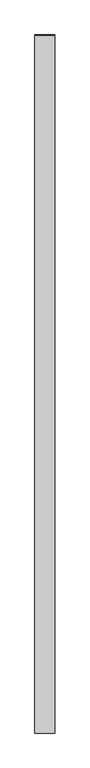
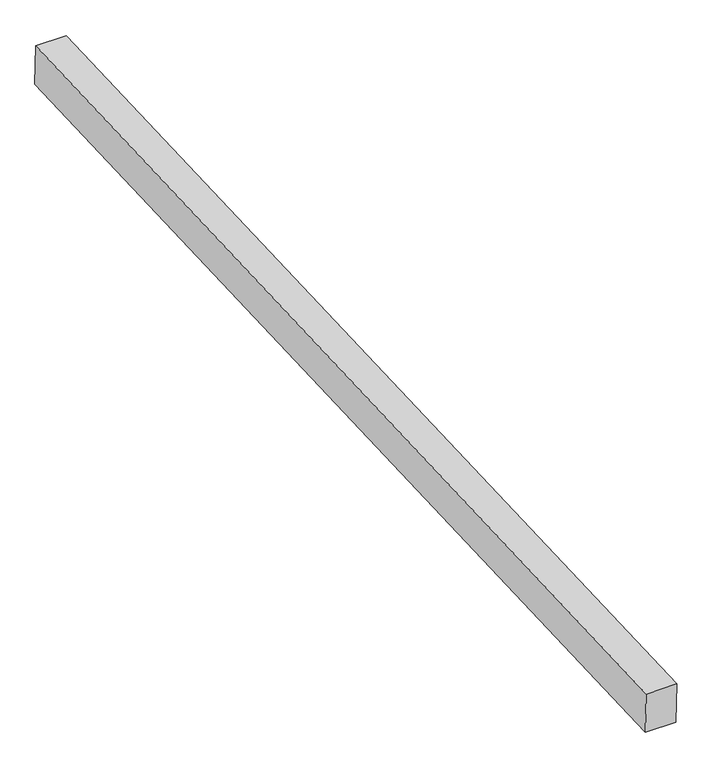
"""IFC4 building model written with IfcOpenShell, lengths in millimetres: proxy geometry, Generic Models 7:Generic Models 1:8:Generic Models 1:8 : Generic Models 7:Generic Models 1:337419:18 : Generic Models 7:Generic Models 1:8:Generic Models 1:8 : Generic Models 7:Generic Models 1:337419:315935."""

import ifcopenshell
import ifcopenshell.guid

model = None  # the IFC model being written
_history = None  # IfcOwnerHistory: only IFC2X3 demands one
_inside = {}  # id of a spatial element -> (the spatial element, [elements in it])
_under = {}  # id of a project, library or spatial element -> (it, [spatial elements below it])
_declared = {}  # id of a project -> (the project, [libraries it declares])
_typed = {}  # id of a type object -> (the type object, [elements of that type])
_made_of = {}  # id of a material, layer set ... -> (it, [elements and type objects made of it])


def new_model(schema):
    """Start an empty IFC model of exactly this schema.

    Asked for "IFC4X3", IfcOpenShell would pick the latest addendum, in which some entities
    have other attributes; the version numbers below select the first issue.
    IFC2X3 requires an IfcOwnerHistory on every rooted entity: one is made here for all.
    """
    global model, _history
    if schema == "IFC4X3":
        model = ifcopenshell.file(schema_version=(4, 3, 0, 0))
    else:
        model = ifcopenshell.file(schema=schema)
    _inside.clear()
    _under.clear()
    _declared.clear()
    _typed.clear()
    _made_of.clear()
    _history = None
    if model.schema == "IFC2X3":
        org = make("IfcOrganization", Name="unknown")
        user = make(
            "IfcPersonAndOrganization",
            ThePerson=make("IfcPerson", FamilyName="unknown"),
            TheOrganization=org,
        )
        app = make(
            "IfcApplication",
            ApplicationDeveloper=org,
            Version="unknown",
            ApplicationFullName="unknown",
            ApplicationIdentifier="unknown",
        )
        _history = make(
            "IfcOwnerHistory",
            OwningUser=user,
            OwningApplication=app,
            ChangeAction="ADDED",
            CreationDate=0,
        )
    return model


def make(cls, **values):
    """One entity of the class cls with the attributes given. An attribute that is None is left unset."""
    return model.create_entity(
        cls, **{name: value for name, value in values.items() if value is not None}
    )


def rooted(cls, **values):
    """An entity with a GlobalId (a new one), such as an element, a storey or a relation."""
    return make(cls, GlobalId=ifcopenshell.guid.new(), OwnerHistory=_history, **values)


def si_unit(unit_type, name, prefix=None):
    """IfcSIUnit, for example si_unit("LENGTHUNIT", "METRE", prefix="MILLI")."""
    return make("IfcSIUnit", UnitType=unit_type, Prefix=prefix, Name=name)


def assignment(units):
    """IfcUnitAssignment: the units of a project."""
    return None if units is None else make("IfcUnitAssignment", Units=units)


def point(xyz):
    """IfcCartesianPoint."""
    return None if xyz is None else make("IfcCartesianPoint", Coordinates=xyz)


def direction(xyz):
    """IfcDirection."""
    return None if xyz is None else make("IfcDirection", DirectionRatios=xyz)


def frame(location, z_axis=None, x_axis=None):
    """IfcAxis2Placement3D, a coordinate frame: its origin and axes. An axis left out is left unset."""
    return make(
        "IfcAxis2Placement3D",
        Location=point(location),
        Axis=direction(z_axis),
        RefDirection=direction(x_axis),
    )


def origin():
    """The frame at (0, 0, 0) with its axes left unset."""
    return frame((0.0, 0.0, 0.0))


def place(relative_to, where):
    """IfcLocalPlacement: puts the frame where relative to a parent placement (None: the world)."""
    return make(
        "IfcLocalPlacement", PlacementRelTo=relative_to, RelativePlacement=where
    )


def context(
    kind, dimensions, precision=None, world=None, true_north=None, identifier=None
):
    """IfcGeometricRepresentationContext, for example the 3D "Model" context."""
    return make(
        "IfcGeometricRepresentationContext",
        ContextIdentifier=identifier,
        ContextType=kind,
        CoordinateSpaceDimension=dimensions,
        Precision=precision,
        WorldCoordinateSystem=world,
        TrueNorth=true_north,
    )


def project(units=None, contexts=None):
    """IfcProject with its units and contexts."""
    return rooted(
        "IfcProject",
        Name="project",
        RepresentationContexts=contexts,
        UnitsInContext=assignment(units),
    )


def spatial(cls, under=None, at=None, **own):
    """A site, building, storey or space (cls), placed at a placement, below another one or the project."""
    s = rooted(cls, ObjectPlacement=at, **own)
    if under is not None:
        _under.setdefault(under.id(), (under, []))[1].append(s)
    return s


def polyline(points):
    """IfcPolyline through the points."""
    return make("IfcPolyline", Points=[point(p) for p in points])


def outline(outer, holes=None, kind="AREA"):
    """IfcArbitraryClosedProfileDef: a profile drawn as a closed curve; with holes, ...WithVoids."""
    if holes is None:
        return make("IfcArbitraryClosedProfileDef", ProfileType=kind, OuterCurve=outer)
    return make(
        "IfcArbitraryProfileDefWithVoids",
        ProfileType=kind,
        OuterCurve=outer,
        InnerCurves=holes,
    )


def extrude(swept, where, along, depth):
    """IfcExtrudedAreaSolid: the profile swept, set in the frame where, extruded along a direction by depth."""
    return make(
        "IfcExtrudedAreaSolid",
        SweptArea=swept,
        Position=where,
        ExtrudedDirection=direction(along),
        Depth=depth,
    )


def shape(context_of_items, identifier, shape_type, items):
    """IfcShapeRepresentation: the items that make up one representation, for example the "Body"."""
    return make(
        "IfcShapeRepresentation",
        ContextOfItems=context_of_items,
        RepresentationIdentifier=identifier,
        RepresentationType=shape_type,
        Items=items,
    )


def source(mapping_origin, context_of_items, identifier, shape_type, items):
    """IfcRepresentationMap: a shape defined once, which mapped items show again and again."""
    return make(
        "IfcRepresentationMap",
        MappingOrigin=mapping_origin,
        MappedRepresentation=shape(context_of_items, identifier, shape_type, items),
    )


def transform(
    local_origin,
    x_axis=None,
    y_axis=None,
    z_axis=None,
    scale=None,
    scale2=None,
    scale3=None,
    uniform=True,
):
    """IfcCartesianTransformationOperator3D, or its non-uniform kind. x_axis, y_axis, z_axis: its Axis1, 2, 3."""
    if uniform:
        return make(
            "IfcCartesianTransformationOperator3D",
            Axis1=direction(x_axis),
            Axis2=direction(y_axis),
            LocalOrigin=point(local_origin),
            Scale=scale,
            Axis3=direction(z_axis),
        )
    return make(
        "IfcCartesianTransformationOperator3DnonUniform",
        Axis1=direction(x_axis),
        Axis2=direction(y_axis),
        LocalOrigin=point(local_origin),
        Scale=scale,
        Axis3=direction(z_axis),
        Scale2=scale2,
        Scale3=scale3,
    )


def mapped(mapping_source, mapping_target):
    """IfcMappedItem: shows the shape of a source again, moved by a transform."""
    return make(
        "IfcMappedItem", MappingSource=mapping_source, MappingTarget=mapping_target
    )


def made_of(thing, what):
    """Note that an element or type object is made of a material, layer set ...; save() writes the relation."""
    if what is not None:
        _made_of.setdefault(what.id(), (what, []))[1].append(thing)
    return thing


def element(
    cls,
    number,
    at=None,
    inside=None,
    cuts=None,
    type_object=None,
    material=None,
    context=None,
    identifier="Body",
    shape_type=None,
    held_by="IfcProductDefinitionShape",
    body=None,
    shapes=None,
    **own,
):
    """One element of the class cls, such as IfcWall. Its Tag is "e" and its number.

    at: its placement. inside: the storey or other place that contains it. cuts: it is an
    opening in that element (IfcRelVoidsElement). A single representation is given by context,
    identifier, shape_type and body (its items); several are given by shapes. held_by: the class
    of the entity that holds the representations. save() writes the other relations.
    """
    e = rooted(cls, Tag="e%d" % number, ObjectPlacement=at, **own)
    if body is not None:
        shapes = [shape(context, identifier, shape_type, body)]
    if shapes is not None:
        e.Representation = make(held_by, Representations=shapes)
    if inside is not None:
        _inside.setdefault(inside.id(), (inside, []))[1].append(e)
    if cuts is not None:
        rooted(
            "IfcRelVoidsElement", RelatingBuildingElement=cuts, RelatedOpeningElement=e
        )
    if type_object is not None:
        _typed.setdefault(type_object.id(), (type_object, []))[1].append(e)
    return made_of(e, material)


def aggregate(whole, parts):
    """IfcRelAggregates: a whole, such as a stair, and the parts it consists of."""
    return rooted("IfcRelAggregates", RelatingObject=whole, RelatedObjects=parts)


def save(model, path):
    """Write the relations noted so far, then the file.

    IfcRelAggregates (storeys below a building ...), IfcRelContainedInSpatialStructure (elements
    in a storey), IfcRelDefinesByType, IfcRelAssociatesMaterial and IfcRelDeclares: one each for
    every whole, place, type object, material and project.
    """
    for whole, parts in _under.values():
        aggregate(whole, parts)
    for where, things in _inside.values():
        rooted(
            "IfcRelContainedInSpatialStructure",
            RelatedElements=things,
            RelatingStructure=where,
        )
    for kind, things in _typed.values():
        rooted("IfcRelDefinesByType", RelatedObjects=things, RelatingType=kind)
    for what, things in _made_of.values():
        rooted("IfcRelAssociatesMaterial", RelatedObjects=things, RelatingMaterial=what)
    for by, libraries in _declared.values():
        rooted("IfcRelDeclares", RelatingContext=by, RelatedDefinitions=libraries)
    model.write(path)


def generic_models_a567c0b8(model_context):
    return source(origin(), model_context, "Body", "SweptSolid", [
        extrude(outline(polyline([(-580626.555738, 3844.0209448), (-575753.6328438, 4047.0593987), (-575746.0659221, 3856.7093942), (-580618.6251193, 3653.6860944), (-580626.555738, 3844.0209448)])), frame((589988.411724, 0.0, 0.0), z_axis=(1.0, 0.0, 0.0), x_axis=(0.0, 1.0, 0.0)), (0.0, 0.0, 1.0), 139.7),
    ])


if __name__ == "__main__":
    model = new_model("IFC4")
    model_context = context("Model", 3, world=origin())
    ifc_project = project(units=[si_unit("LENGTHUNIT", "METRE", prefix="MILLI")], contexts=[model_context])
    site = spatial("IfcSite", under=ifc_project)
    building = spatial("IfcBuilding", under=site)
    placement = place(None, origin())
    generic_models_shape = generic_models_a567c0b8(model_context)
    element("IfcBuildingElementProxy", 1, Name="Generic Models 7:Generic Models 1:8:Generic Models 1:8 : Generic Models 7:Generic Models 1:337419:18 : Generic Models 7:Generic Models 1:8:Generic Models 1:8 : Generic Models 7:Generic Models 1:337419:315935", ObjectType="Generic Models 7:Generic Models 1:8:Generic Models 1:8 : Generic Models 7:Generic Models 1:337419:18 : Generic Models 7:Generic Models 1:8:Generic Models 1:8 : Generic Models 7:Generic Models 1:337419:315935", at=placement, inside=building, context=model_context, shape_type="MappedRepresentation", body=[
        mapped(generic_models_shape, transform((0.0, 0.0, 0.0), x_axis=(1.0, 0.0, 0.0), y_axis=(0.0, 1.0, 0.0), z_axis=(0.0, 0.0, 1.0))),
    ])
    save(model, "model.ifc")

# Revit data of these elements
# Type "Generic Models 7:Generic Models 1:8:Generic Models 1:8 : Generic Models 7:Generic Models 1:337419:18 : Generic Models 7:Generic Models 1:8:Generic Models 1:8 : Generic Models 7:Generic Models 1:337419:315935"
#   NameOverride = "Generic Models 7:Generic Models 1:8:Generic Models 1:8 : Generic Models 7:Generic Models 1:337419:315935"
#   ObjectTypeOverride = "Generic Models 1:8 : Generic Models 7:Generic Models 1:337419"
#   Reference = "Generic Models 1"
#   Tag = "315935"
# Element 1 (IfcBuildingElementProxy, "Generic Models 7:Generic Models 1:8:Generic Models 1:8 : Generic Models 7:Generic Models 1:337419:18 : Generic Models 7:Generic Models 1:8:Generic Models 1:8 : Generic Models 7:Generic Models 1:337419:315935")
#   Materials on its faces: "5 1/2\" X 7 1/2\" EXTERIOR GRADE GLULAM BEAMS"
# Materials
#   "5 1/2\" X 7 1/2\" EXTERIOR GRADE GLULAM BEAMS": class "Wood", colour RGB 183 134 68, transparency 0, Keynote = "M06181300.01", Description = "Pinus Echinata", Cost = 0
